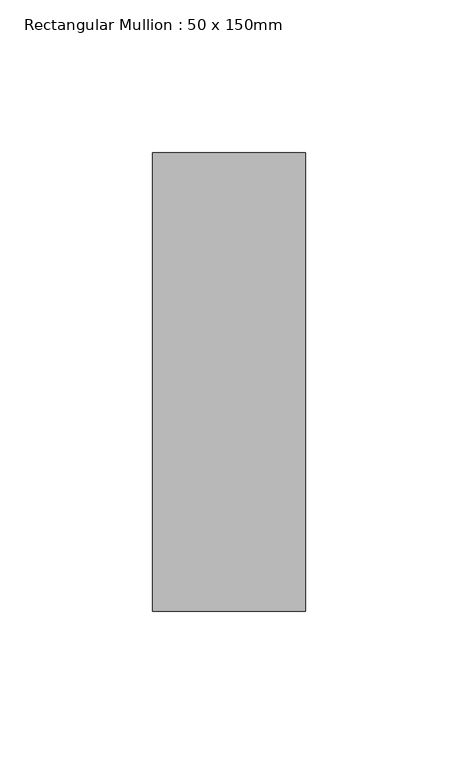
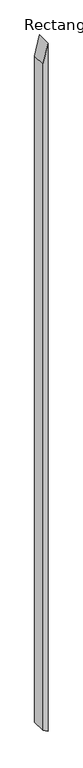
"""IFC4 building model written with IfcOpenShell, lengths in millimetres: member geometry, Rectangular Mullion : 50 x 150mm."""

from ifc_helpers import new_model, si_unit, frame, origin, place, context, project, spatial, polyline, outline, extrude, source, transform, mapped, element, save


def rectangular_mullion_50_x_150mm_45e6ae42(model_context):
    return source(origin(), model_context, "Body", "SweptSolid", [
        extrude(outline(polyline([(0.0, 0.0), (-213.5028682, -50.0), (-7489.7328456, -50.0), (-7519.6193703, 0.0), (0.0, 0.0)])), frame((0.0, -75.0, 0.0), z_axis=(0.0, 1.0, 0.0), x_axis=(0.0, 0.0, 1.0)), (0.0, 0.0, 1.0), 150.0),
    ])


if __name__ == "__main__":
    model = new_model("IFC4")
    model_context = context("Model", 3, world=origin())
    ifc_project = project(units=[si_unit("LENGTHUNIT", "METRE", prefix="MILLI")], contexts=[model_context])
    site = spatial("IfcSite", under=ifc_project)
    building = spatial("IfcBuilding", under=site)
    placement = place(None, origin())
    rectangular_mullion_50_x_150mm_shape = rectangular_mullion_50_x_150mm_45e6ae42(model_context)
    element("IfcMember", 1, ObjectType="Rectangular Mullion : 50 x 150mm", at=placement, inside=building, context=model_context, shape_type="MappedRepresentation", body=[
        mapped(rectangular_mullion_50_x_150mm_shape, transform((0.0, 0.0, 0.0), x_axis=(1.0, 0.0, 0.0), y_axis=(0.0, 1.0, 0.0), z_axis=(0.0, 0.0, 1.0))),
    ])
    save(model, "model.ifc")

# Revit data of these elements
# Type "Rectangular Mullion : 50 x 150mm"
#   built-in parameter 1007304 = 0.492126 (stored number, unit not read)
#   built-in parameter 1007301 = 0.082021 (stored number, unit not read)
#   built-in parameter 1007300 = 0.082021 (stored number, unit not read)
# Element 1 (IfcMember, "Rectangular Mullion : 50 x 150mm")
#   Materials on its faces: "Metal - Aluminium"
# Materials
#   "Metal - Aluminium": class "Metal", colour RGB 247 247 247, transparency 0
